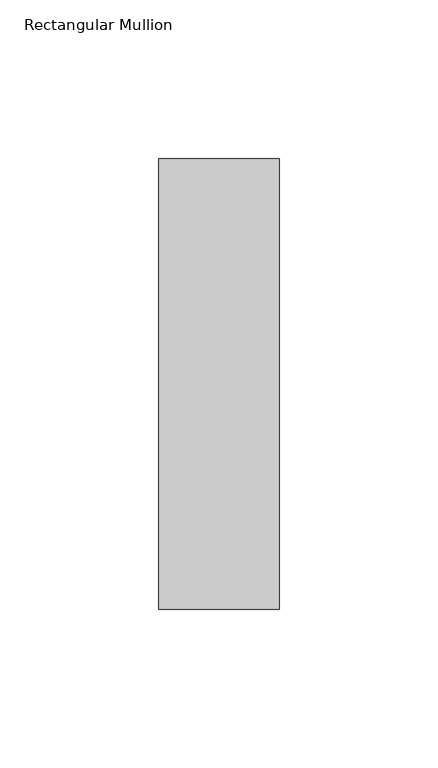
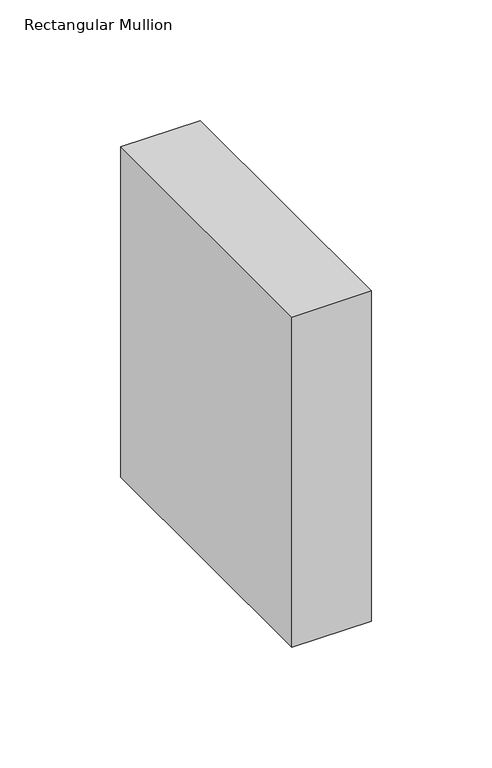
"""IFC4 building model written with IfcOpenShell, lengths in millimetres: member geometry, Rectangular Mullion : NLRS_21_CWM_hsb-regel 38x142_gen_rsf."""

import ifcopenshell
import ifcopenshell.guid

model = None  # the IFC model being written
_history = None  # IfcOwnerHistory: only IFC2X3 demands one
_inside = {}  # id of a spatial element -> (the spatial element, [elements in it])
_under = {}  # id of a project, library or spatial element -> (it, [spatial elements below it])
_declared = {}  # id of a project -> (the project, [libraries it declares])
_typed = {}  # id of a type object -> (the type object, [elements of that type])
_made_of = {}  # id of a material, layer set ... -> (it, [elements and type objects made of it])


def new_model(schema):
    """Start an empty IFC model of exactly this schema.

    Asked for "IFC4X3", IfcOpenShell would pick the latest addendum, in which some entities
    have other attributes; the version numbers below select the first issue.
    IFC2X3 requires an IfcOwnerHistory on every rooted entity: one is made here for all.
    """
    global model, _history
    if schema == "IFC4X3":
        model = ifcopenshell.file(schema_version=(4, 3, 0, 0))
    else:
        model = ifcopenshell.file(schema=schema)
    _inside.clear()
    _under.clear()
    _declared.clear()
    _typed.clear()
    _made_of.clear()
    _history = None
    if model.schema == "IFC2X3":
        org = make("IfcOrganization", Name="unknown")
        user = make(
            "IfcPersonAndOrganization",
            ThePerson=make("IfcPerson", FamilyName="unknown"),
            TheOrganization=org,
        )
        app = make(
            "IfcApplication",
            ApplicationDeveloper=org,
            Version="unknown",
            ApplicationFullName="unknown",
            ApplicationIdentifier="unknown",
        )
        _history = make(
            "IfcOwnerHistory",
            OwningUser=user,
            OwningApplication=app,
            ChangeAction="ADDED",
            CreationDate=0,
        )
    return model


def make(cls, **values):
    """One entity of the class cls with the attributes given. An attribute that is None is left unset."""
    return model.create_entity(
        cls, **{name: value for name, value in values.items() if value is not None}
    )


def rooted(cls, **values):
    """An entity with a GlobalId (a new one), such as an element, a storey or a relation."""
    return make(cls, GlobalId=ifcopenshell.guid.new(), OwnerHistory=_history, **values)


def si_unit(unit_type, name, prefix=None):
    """IfcSIUnit, for example si_unit("LENGTHUNIT", "METRE", prefix="MILLI")."""
    return make("IfcSIUnit", UnitType=unit_type, Prefix=prefix, Name=name)


def assignment(units):
    """IfcUnitAssignment: the units of a project."""
    return None if units is None else make("IfcUnitAssignment", Units=units)


def point(xyz):
    """IfcCartesianPoint."""
    return None if xyz is None else make("IfcCartesianPoint", Coordinates=xyz)


def direction(xyz):
    """IfcDirection."""
    return None if xyz is None else make("IfcDirection", DirectionRatios=xyz)


def frame(location, z_axis=None, x_axis=None):
    """IfcAxis2Placement3D, a coordinate frame: its origin and axes. An axis left out is left unset."""
    return make(
        "IfcAxis2Placement3D",
        Location=point(location),
        Axis=direction(z_axis),
        RefDirection=direction(x_axis),
    )


def origin():
    """The frame at (0, 0, 0) with its axes left unset."""
    return frame((0.0, 0.0, 0.0))


def place(relative_to, where):
    """IfcLocalPlacement: puts the frame where relative to a parent placement (None: the world)."""
    return make(
        "IfcLocalPlacement", PlacementRelTo=relative_to, RelativePlacement=where
    )


def context(
    kind, dimensions, precision=None, world=None, true_north=None, identifier=None
):
    """IfcGeometricRepresentationContext, for example the 3D "Model" context."""
    return make(
        "IfcGeometricRepresentationContext",
        ContextIdentifier=identifier,
        ContextType=kind,
        CoordinateSpaceDimension=dimensions,
        Precision=precision,
        WorldCoordinateSystem=world,
        TrueNorth=true_north,
    )


def project(units=None, contexts=None):
    """IfcProject with its units and contexts."""
    return rooted(
        "IfcProject",
        Name="project",
        RepresentationContexts=contexts,
        UnitsInContext=assignment(units),
    )


def spatial(cls, under=None, at=None, **own):
    """A site, building, storey or space (cls), placed at a placement, below another one or the project."""
    s = rooted(cls, ObjectPlacement=at, **own)
    if under is not None:
        _under.setdefault(under.id(), (under, []))[1].append(s)
    return s


def polyline(points):
    """IfcPolyline through the points."""
    return make("IfcPolyline", Points=[point(p) for p in points])


def outline(outer, holes=None, kind="AREA"):
    """IfcArbitraryClosedProfileDef: a profile drawn as a closed curve; with holes, ...WithVoids."""
    if holes is None:
        return make("IfcArbitraryClosedProfileDef", ProfileType=kind, OuterCurve=outer)
    return make(
        "IfcArbitraryProfileDefWithVoids",
        ProfileType=kind,
        OuterCurve=outer,
        InnerCurves=holes,
    )


def extrude(swept, where, along, depth):
    """IfcExtrudedAreaSolid: the profile swept, set in the frame where, extruded along a direction by depth."""
    return make(
        "IfcExtrudedAreaSolid",
        SweptArea=swept,
        Position=where,
        ExtrudedDirection=direction(along),
        Depth=depth,
    )


def shape(context_of_items, identifier, shape_type, items):
    """IfcShapeRepresentation: the items that make up one representation, for example the "Body"."""
    return make(
        "IfcShapeRepresentation",
        ContextOfItems=context_of_items,
        RepresentationIdentifier=identifier,
        RepresentationType=shape_type,
        Items=items,
    )


def source(mapping_origin, context_of_items, identifier, shape_type, items):
    """IfcRepresentationMap: a shape defined once, which mapped items show again and again."""
    return make(
        "IfcRepresentationMap",
        MappingOrigin=mapping_origin,
        MappedRepresentation=shape(context_of_items, identifier, shape_type, items),
    )


def transform(
    local_origin,
    x_axis=None,
    y_axis=None,
    z_axis=None,
    scale=None,
    scale2=None,
    scale3=None,
    uniform=True,
):
    """IfcCartesianTransformationOperator3D, or its non-uniform kind. x_axis, y_axis, z_axis: its Axis1, 2, 3."""
    if uniform:
        return make(
            "IfcCartesianTransformationOperator3D",
            Axis1=direction(x_axis),
            Axis2=direction(y_axis),
            LocalOrigin=point(local_origin),
            Scale=scale,
            Axis3=direction(z_axis),
        )
    return make(
        "IfcCartesianTransformationOperator3DnonUniform",
        Axis1=direction(x_axis),
        Axis2=direction(y_axis),
        LocalOrigin=point(local_origin),
        Scale=scale,
        Axis3=direction(z_axis),
        Scale2=scale2,
        Scale3=scale3,
    )


def mapped(mapping_source, mapping_target):
    """IfcMappedItem: shows the shape of a source again, moved by a transform."""
    return make(
        "IfcMappedItem", MappingSource=mapping_source, MappingTarget=mapping_target
    )


def made_of(thing, what):
    """Note that an element or type object is made of a material, layer set ...; save() writes the relation."""
    if what is not None:
        _made_of.setdefault(what.id(), (what, []))[1].append(thing)
    return thing


def element(
    cls,
    number,
    at=None,
    inside=None,
    cuts=None,
    type_object=None,
    material=None,
    context=None,
    identifier="Body",
    shape_type=None,
    held_by="IfcProductDefinitionShape",
    body=None,
    shapes=None,
    **own,
):
    """One element of the class cls, such as IfcWall. Its Tag is "e" and its number.

    at: its placement. inside: the storey or other place that contains it. cuts: it is an
    opening in that element (IfcRelVoidsElement). A single representation is given by context,
    identifier, shape_type and body (its items); several are given by shapes. held_by: the class
    of the entity that holds the representations. save() writes the other relations.
    """
    e = rooted(cls, Tag="e%d" % number, ObjectPlacement=at, **own)
    if body is not None:
        shapes = [shape(context, identifier, shape_type, body)]
    if shapes is not None:
        e.Representation = make(held_by, Representations=shapes)
    if inside is not None:
        _inside.setdefault(inside.id(), (inside, []))[1].append(e)
    if cuts is not None:
        rooted(
            "IfcRelVoidsElement", RelatingBuildingElement=cuts, RelatedOpeningElement=e
        )
    if type_object is not None:
        _typed.setdefault(type_object.id(), (type_object, []))[1].append(e)
    return made_of(e, material)


def aggregate(whole, parts):
    """IfcRelAggregates: a whole, such as a stair, and the parts it consists of."""
    return rooted("IfcRelAggregates", RelatingObject=whole, RelatedObjects=parts)


def save(model, path):
    """Write the relations noted so far, then the file.

    IfcRelAggregates (storeys below a building ...), IfcRelContainedInSpatialStructure (elements
    in a storey), IfcRelDefinesByType, IfcRelAssociatesMaterial and IfcRelDeclares: one each for
    every whole, place, type object, material and project.
    """
    for whole, parts in _under.values():
        aggregate(whole, parts)
    for where, things in _inside.values():
        rooted(
            "IfcRelContainedInSpatialStructure",
            RelatedElements=things,
            RelatingStructure=where,
        )
    for kind, things in _typed.values():
        rooted("IfcRelDefinesByType", RelatedObjects=things, RelatingType=kind)
    for what, things in _made_of.values():
        rooted("IfcRelAssociatesMaterial", RelatedObjects=things, RelatingMaterial=what)
    for by, libraries in _declared.values():
        rooted("IfcRelDeclares", RelatingContext=by, RelatedDefinitions=libraries)
    model.write(path)


def rectangular_mullion_c6f7c22d(model_context):
    return source(origin(), model_context, "Body", "SweptSolid", [
        extrude(outline(polyline([(-38.0, -71.0), (-38.0, 71.0), (0.0, 71.0), (0.0, -71.0), (-38.0, -71.0)])), frame((0.0, 0.0, -167.1558939), z_axis=(0.0, 0.0, 1.0), x_axis=(1.0, 0.0, 0.0)), (0.0, 0.0, 1.0), 167.1558939),
    ])


if __name__ == "__main__":
    model = new_model("IFC4")
    model_context = context("Model", 3, world=origin())
    ifc_project = project(units=[si_unit("LENGTHUNIT", "METRE", prefix="MILLI")], contexts=[model_context])
    site = spatial("IfcSite", under=ifc_project)
    building = spatial("IfcBuilding", under=site)
    placement = place(None, origin())
    rectangular_mullion_shape = rectangular_mullion_c6f7c22d(model_context)
    element("IfcMember", 1, ObjectType="Rectangular Mullion : NLRS_21_CWM_hsb-regel 38x142_gen_rsf", at=placement, inside=building, context=model_context, shape_type="MappedRepresentation", body=[
        mapped(rectangular_mullion_shape, transform((0.0, 0.0, 0.0), x_axis=(1.0, 0.0, 0.0), y_axis=(0.0, 1.0, 0.0), z_axis=(0.0, 0.0, 1.0))),
    ])
    save(model, "model.ifc")

# Revit data of these elements
# Type "Rectangular Mullion : NLRS_21_CWM_hsb-regel 38x142_gen_rsf"
#   Export Type to IFC As = "IfcWall"
#   Type IfcGUID = "07M7mRoiH1CR8m_RSKIwpF"
#   Assembly Code = "21.10"
#   built-in parameter 1007322 = 0.465879 (stored number, unit not read)
#   built-in parameter 1007321 = 0.062336 (stored number, unit not read)
#   built-in parameter 1007320 = 0.062336 (stored number, unit not read)
# Element 1 (IfcMember, "Rectangular Mullion : NLRS_21_CWM_hsb-regel 38x142_gen_rsf")
#   Materials on its faces: "NLRS_i2_hout naaldhout vuren_gen_rsf"
# Materials
#   "NLRS_i2_hout naaldhout vuren_gen_rsf": class "I - Hout", colour RGB 234 199 147, transparency 0, Keynote = "i2", Manufacturer = "Revit Standards Foundation", URL = "www.revitstandards.org", Description = "hout vuren", Cost = 0
